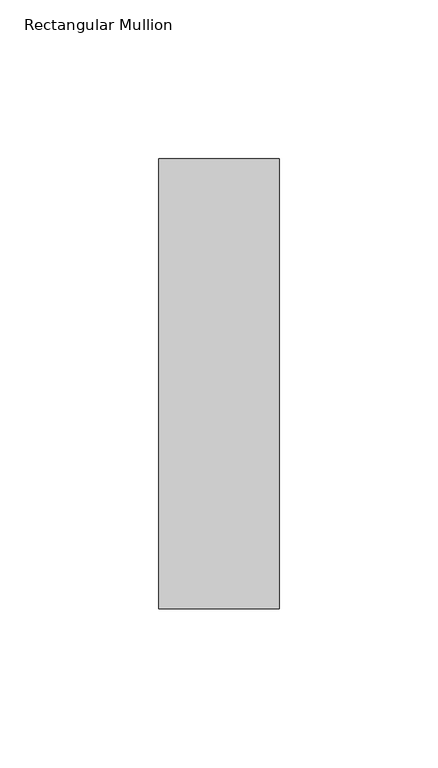
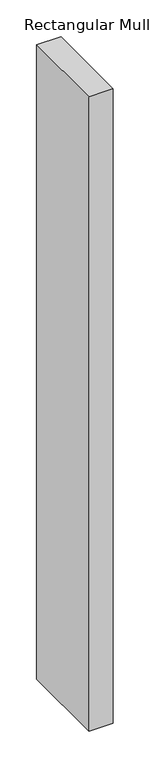
"""IFC4 building model written with IfcOpenShell, lengths in millimetres: member geometry, Rectangular Mullion : NLRS_21_CWM_hsb-regel 38x142_gen_rsf."""

from ifc_helpers import new_model, si_unit, frame, origin, place, context, project, spatial, polyline, outline, extrude, source, transform, mapped, element, save


def rectangular_mullion_1165df42(model_context):
    return source(origin(), model_context, "Body", "SweptSolid", [
        extrude(outline(polyline([(-38.0, -71.0), (-38.0, 71.0), (0.0, 71.0), (0.0, -71.0), (-38.0, -71.0)])), frame((0.0, 0.0, -1050.0), z_axis=(0.0, 0.0, 1.0), x_axis=(1.0, 0.0, 0.0)), (0.0, 0.0, 1.0), 1050.0),
    ])


if __name__ == "__main__":
    model = new_model("IFC4")
    model_context = context("Model", 3, world=origin())
    ifc_project = project(units=[si_unit("LENGTHUNIT", "METRE", prefix="MILLI")], contexts=[model_context])
    site = spatial("IfcSite", under=ifc_project)
    building = spatial("IfcBuilding", under=site)
    placement = place(None, origin())
    rectangular_mullion_shape = rectangular_mullion_1165df42(model_context)
    element("IfcMember", 1, ObjectType="Rectangular Mullion : NLRS_21_CWM_hsb-regel 38x142_gen_rsf", at=placement, inside=building, context=model_context, shape_type="MappedRepresentation", body=[
        mapped(rectangular_mullion_shape, transform((0.0, 0.0, 0.0), x_axis=(1.0, 0.0, 0.0), y_axis=(0.0, 1.0, 0.0), z_axis=(0.0, 0.0, 1.0))),
    ])
    save(model, "model.ifc")

# Revit data of these elements
# Type "Rectangular Mullion : NLRS_21_CWM_hsb-regel 38x142_gen_rsf"
#   Export Type to IFC As = "IfcWall"
#   Type IfcGUID = "07M7mRoiH1CR8m_RSKIwpF"
#   Assembly Code = "21.10"
#   built-in parameter 1007322 = 0.465879 (stored number, unit not read)
#   built-in parameter 1007321 = 0.062336 (stored number, unit not read)
#   built-in parameter 1007320 = 0.062336 (stored number, unit not read)
# Element 1 (IfcMember, "Rectangular Mullion : NLRS_21_CWM_hsb-regel 38x142_gen_rsf")
#   Materials on its faces: "NLRS_i2_hout naaldhout vuren_gen_rsf"
# Materials
#   "NLRS_i2_hout naaldhout vuren_gen_rsf": class "I - Hout", colour RGB 234 199 147, transparency 0, Keynote = "i2", Manufacturer = "Revit Standards Foundation", URL = "www.revitstandards.org", Description = "hout vuren", Cost = 0
